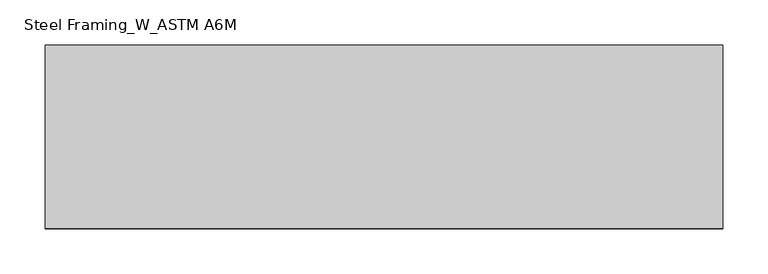
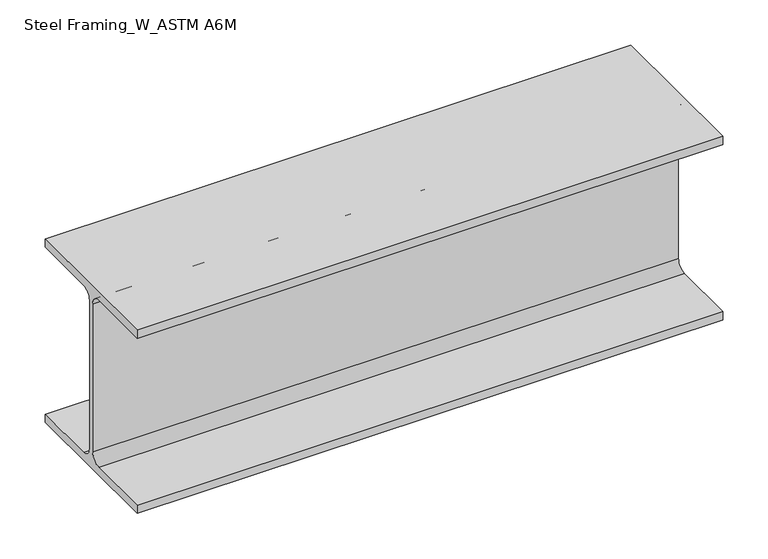
"""IFC4 building model written with IfcOpenShell, lengths in millimetres: beam geometry, Steel Framing_W_ASTM A6M : H_SB_AR_S02_W250x49.1_RCG1."""

from ifc_helpers import new_model, si_unit, point, frame, frame_2d, origin, place, context, project, spatial, polyline, circle_curve, trimmed, segment, composite_curve, outline, extrude, source, transform, mapped, element, save


def steel_framing_w_astm_a6m_d7cd949d(model_context):
    return source(origin(), model_context, "Body", "SweptSolid", [
        extrude(outline(composite_curve([segment(polyline([(101.0, -112.5), (101.0, -123.5), (-101.0, -123.5), (-101.0, -112.5), (-16.385, -112.5)]), True, "CONTINUOUS"), segment(trimmed(circle_curve(frame_2d((-16.385, -99.8)), 12.7), [point((-16.385, -112.5))], [point((-3.685, -99.8))], True, "CARTESIAN"), True, "CONTINUOUS"), segment(polyline([(-3.685, -99.8), (-3.685, 99.8)]), True, "CONTINUOUS"), segment(trimmed(circle_curve(frame_2d((-16.385, 99.8)), 12.7), [point((-3.685, 99.8))], [point((-16.385, 112.5))], True, "CARTESIAN"), True, "CONTINUOUS"), segment(polyline([(-16.385, 112.5), (-101.0, 112.5), (-101.0, 123.5), (101.0, 123.5), (101.0, 112.5), (16.385, 112.5)]), True, "CONTINUOUS"), segment(trimmed(circle_curve(frame_2d((16.385, 99.8)), 12.7), [point((16.385, 112.5))], [point((3.685, 99.8))], True, "CARTESIAN"), True, "CONTINUOUS"), segment(polyline([(3.685, 99.8), (3.685, -99.8)]), True, "CONTINUOUS"), segment(trimmed(circle_curve(frame_2d((16.385, -99.8)), 12.7), [point((3.685, -99.8))], [point((16.385, -112.5))], True, "CARTESIAN"), True, "CONTINUOUS"), segment(polyline([(16.385, -112.5), (101.0, -112.5)]), True, "CONTINUOUS")], self_intersect=False)), frame((-236.55, 0.0, 0.0), z_axis=(1.0, 0.0, 0.0), x_axis=(0.0, 1.0, 0.0)), (0.0, 0.0, 1.0), 745.2),
    ])


if __name__ == "__main__":
    model = new_model("IFC4")
    model_context = context("Model", 3, world=origin())
    ifc_project = project(units=[si_unit("LENGTHUNIT", "METRE", prefix="MILLI")], contexts=[model_context])
    site = spatial("IfcSite", under=ifc_project)
    building = spatial("IfcBuilding", under=site)
    placement = place(None, origin())
    steel_framing_w_astm_a6m_shape = steel_framing_w_astm_a6m_d7cd949d(model_context)
    element("IfcBeam", 1, ObjectType="Steel Framing_W_ASTM A6M : H_SB_AR_S02_W250x49.1_RCG1", at=placement, inside=building, context=model_context, shape_type="MappedRepresentation", body=[
        mapped(steel_framing_w_astm_a6m_shape, transform((0.0, 0.0, 0.0), x_axis=(1.0, 0.0, 0.0), y_axis=(0.0, 1.0, 0.0), z_axis=(0.0, 0.0, 1.0))),
    ])
    save(model, "model.ifc")

# Revit data of these elements
# Type "Steel Framing_W_ASTM A6M : H_SB_AR_S02_W250x49.1_RCG1"
#   Type Mark = "RCG1"
#   Section Name Key = "W10x33"
#   Width = 20.2 cm
#   Web Thickness = 0.737 cm
#   Web Fillet = 1.27 cm
#   Warping Constant = 212000.0 cm⁶
#   Torsional Moment of Inertia = 24.30 cm⁴
#   Section Area = 62.6 cm²
#   Plastic Modulus weak axis = 229.0 cm³
#   Plastic Modulus strong axis = 636.0 cm³
#   Perimeter = 1.27 m²/m
#   Nominal Weight = 49.10 kgf/m
#   Moment of Inertia weak axis = 1520.00 cm⁴
#   Moment of Inertia strong axis = 7120.00 cm⁴
#   Height = 24.7 cm
#   Flange Thickness = 1.1 cm
#   Elastic Modulus weak axis = 151.0 cm³
#   Elastic Modulus strong axis = 574.0 cm³
#   Centroid Vertical = 12.35 cm
#   Centroid Horizontal = 10.1 cm
#   Length [instance default] = 1500 mm
#   Structural Material [instance default] = Steel, 45-345
#   Bolt Spacing = 0
#   Assembly Code = ""
# Element 1 (IfcBeam, "Steel Framing_W_ASTM A6M : H_SB_AR_S02_W250x49.1_RCG1")
#   Materials on its faces: "Steel, 45-345"
# Materials
#   "Steel, 45-345": class "Metal", colour RGB 189 187 185, transparency 0, Description = "Steel 345 MPa", Cost = 0
